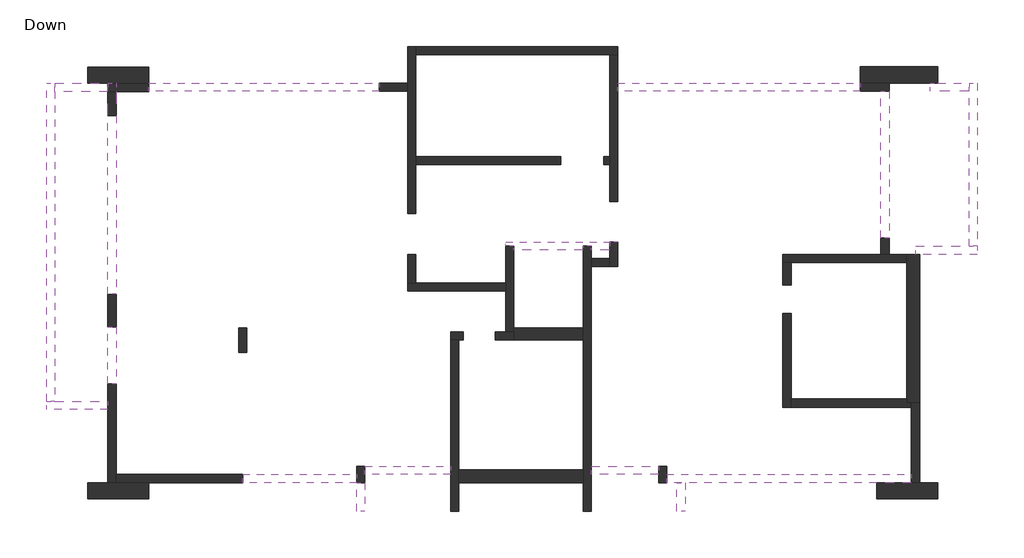
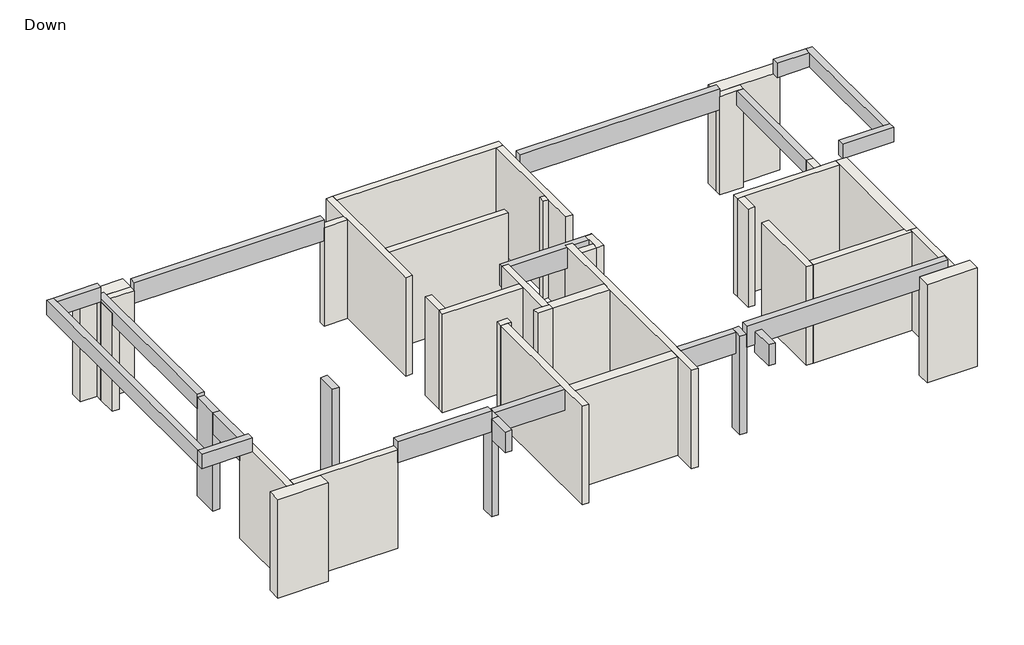
# One storey: 33 walls, 18 beams, 4 columns.
# Revit data of these elements (continued)
# Element 23 (IfcWall, "20") (continued)
#   SOFiSTiK_AMG_Comments = ""
#   Top Offset = 0 cm
#   Base Offset = 0 cm
#   wall height = 310 cm
#   SOFiSTiK_AMG_Scheduled = yes
#   SOFiSTiK_AMG_Adjusted = yes
#   Phase Created = New Construction
#   Base Constraint = Down
#   Top Constraint = Typical Floor
#   Materials on its faces: "Concrete"
# Element 24 (IfcWall, "20")
#   Comments = ""
#   Mark = "W6"
#   SOFiSTiK_EdgeZones = "W6"
#   SOFiSTiK_AMG_Comments = ""
#   Top Offset = 0 cm
#   Base Offset = 0 cm
#   wall height = 310 cm
#   SOFiSTiK_AMG_Scheduled = yes
#   SOFiSTiK_AMG_Adjusted = yes
#   Phase Created = New Construction
#   Base Constraint = Down
#   Top Constraint = Typical Floor
#   Materials on its faces: "Concrete"
# Element 25 (IfcWall, "20")
#   Comments = ""
#   Mark = "W7"
#   SOFiSTiK_EdgeZones = "W7"
#   SOFiSTiK_AMG_Comments = ""
#   Top Offset = 0 cm
#   Base Offset = 0 cm
#   wall height = 310 cm
#   SOFiSTiK_AMG_Scheduled = yes
#   SOFiSTiK_AMG_Adjusted = yes
#   Phase Created = New Construction
#   Base Constraint = Down
#   Top Constraint = Typical Floor
#   Materials on its faces: "Concrete"
# Element 26 (IfcWall, "20")
#   Comments = ""
#   Mark = "W8"
#   SOFiSTiK_EdgeZones = "W8"
#   SOFiSTiK_AMG_Comments = ""
#   Top Offset = 0 cm
#   Base Offset = 0 cm
#   wall height = 310 cm
#   SOFiSTiK_AMG_Scheduled = yes
#   SOFiSTiK_AMG_Adjusted = yes
#   Phase Created = New Construction
#   Base Constraint = Down
#   Top Constraint = Typical Floor
#   Materials on its faces: "Concrete"
# Element 27 (IfcWall, "20")
#   Comments = ""
#   Mark = "W9"
#   SOFiSTiK_EdgeZones = "W9"
#   SOFiSTiK_AMG_Comments = ""
#   Top Offset = 0 cm
#   Base Offset = 0 cm
#   wall height = 310 cm
#   SOFiSTiK_AMG_Scheduled = yes
#   SOFiSTiK_AMG_Adjusted = yes
#   Phase Created = New Construction
#   Base Constraint = Down
#   Top Constraint = Typical Floor
#   Materials on its faces: "Concrete"
# Element 28 (IfcWall, "20")
#   Comments = ""
#   Mark = "W10"
#   SOFiSTiK_EdgeZones = "W10"
#   SOFiSTiK_AMG_Comments = ""
#   Top Offset = 0 cm
#   Base Offset = 0 cm
#   wall height = 310 cm
#   SOFiSTiK_AMG_Scheduled = yes
#   SOFiSTiK_AMG_Adjusted = yes
#   Phase Created = New Construction
#   Base Constraint = Down
#   Top Constraint = Typical Floor
#   Materials on its faces: "Concrete"
# Element 29 (IfcWall, "20")
#   Comments = ""
#   Mark = "W11"
#   SOFiSTiK_EdgeZones = "W11"
#   SOFiSTiK_AMG_Comments = ""
#   Top Offset = 0 cm
#   Base Offset = 0 cm
#   wall height = 310 cm
#   SOFiSTiK_AMG_Scheduled = yes
#   SOFiSTiK_AMG_Adjusted = yes
#   Phase Created = New Construction
#   Base Constraint = Down
#   Top Constraint = Typical Floor
#   Materials on its faces: "Concrete"
# Element 30 (IfcWall, "20")
#   Comments = ""
#   Mark = "W12"
#   SOFiSTiK_EdgeZones = "W12"
#   SOFiSTiK_AMG_Comments = ""
#   Top Offset = 0 cm
#   Base Offset = 0 cm
#   wall height = 310 cm
#   SOFiSTiK_AMG_Scheduled = yes
#   SOFiSTiK_AMG_Adjusted = yes
#   Phase Created = New Construction
#   Base Constraint = Down
#   Top Constraint = Typical Floor
#   Materials on its faces: "Concrete"
# Element 31 (IfcWall, "20")
#   Comments = ""
#   Mark = "W13"
#   SOFiSTiK_EdgeZones = "W13"
#   SOFiSTiK_AMG_Comments = ""
#   Top Offset = 0 cm
#   Base Offset = 0 cm
#   wall height = 310 cm
#   SOFiSTiK_AMG_Scheduled = yes
#   SOFiSTiK_AMG_Adjusted = yes
#   Phase Created = New Construction
#   Base Constraint = Down
#   Top Constraint = Typical Floor
#   Materials on its faces: "Concrete"
# Element 32 (IfcWall, "20")
#   Comments = ""
#   Mark = "W14"
#   SOFiSTiK_EdgeZones = "W14"
#   SOFiSTiK_AMG_Comments = ""
#   Top Offset = 0 cm
#   Base Offset = 0 cm
#   wall height = 310 cm
#   SOFiSTiK_AMG_Scheduled = yes
#   SOFiSTiK_AMG_Adjusted = yes
#   Phase Created = New Construction
#   Base Constraint = Down
#   Top Constraint = Typical Floor
#   Materials on its faces: "Concrete"
# Element 33 (IfcWall, "20")
#   Comments = ""
#   Mark = "W16"
#   SOFiSTiK_EdgeZones = "W16"
#   SOFiSTiK_AMG_Comments = ""
#   Top Offset = 0 cm
#   Base Offset = 0 cm
#   wall height = 310 cm
#   SOFiSTiK_AMG_Scheduled = yes
#   SOFiSTiK_AMG_Adjusted = yes
#   Phase Created = New Construction
#   Base Constraint = Down
#   Top Constraint = Typical Floor
#   Materials on its faces: "Concrete"
# Element 34 (IfcWall, "20")
#   Comments = ""
#   Mark = "W17"
#   SOFiSTiK_EdgeZones = "W17"
#   SOFiSTiK_AMG_Comments = ""
#   Top Offset = 0 cm
#   Base Offset = 0 cm
#   wall height = 310 cm
#   SOFiSTiK_AMG_Scheduled = yes
#   SOFiSTiK_AMG_Adjusted = yes
#   Phase Created = New Construction
#   Base Constraint = Down
#   Top Constraint = Typical Floor
#   Materials on its faces: "Concrete"
# Element 35 (IfcWall, "20")
#   Comments = ""
#   Mark = "W18"
#   SOFiSTiK_EdgeZones = "W18"
#   SOFiSTiK_AMG_Comments = ""
#   Top Offset = 0 cm
#   Base Offset = 0 cm
#   wall height = 310 cm
#   SOFiSTiK_AMG_Scheduled = yes
#   SOFiSTiK_AMG_Adjusted = yes
#   Phase Created = New Construction
#   Base Constraint = Down
#   Top Constraint = Typical Floor
#   Materials on its faces: "Concrete"
# Element 36 (IfcWall, "20")
#   Comments = ""
#   Mark = "W19"
#   SOFiSTiK_EdgeZones = "W19"
#   SOFiSTiK_AMG_Comments = ""
#   Top Offset = 0 cm
#   Base Offset = 0 cm
#   wall height = 310 cm
#   SOFiSTiK_AMG_Scheduled = yes
#   SOFiSTiK_AMG_Adjusted = yes
#   Phase Created = New Construction
#   Base Constraint = Down
#   Top Constraint = Typical Floor
#   Materials on its faces: "Concrete"
# Element 37 (IfcWall, "20")
#   Comments = ""
#   Mark = "W20"
#   SOFiSTiK_EdgeZones = "W20"
#   SOFiSTiK_AMG_Comments = ""
#   Top Offset = 0 cm
#   Base Offset = 0 cm
#   wall height = 310 cm
#   SOFiSTiK_AMG_Scheduled = yes
#   SOFiSTiK_AMG_Adjusted = yes
#   Phase Created = New Construction
#   Base Constraint = Down
#   Top Constraint = Typical Floor
#   Materials on its faces: "Concrete"
# Element 38 (IfcWall, "20")
#   Comments = ""
#   Mark = "W21"
#   SOFiSTiK_EdgeZones = "W21"
#   SOFiSTiK_AMG_Comments = ""
#   Top Offset = 0 cm
#   Base Offset = 0 cm
#   wall height = 310 cm
#   SOFiSTiK_AMG_Scheduled = yes
#   SOFiSTiK_AMG_Adjusted = yes
#   Phase Created = New Construction
#   Base Constraint = Down
#   Top Constraint = Typical Floor
#   Materials on its faces: "Concrete"
# Element 39 (IfcWall, "20")
#   Comments = ""
#   Mark = "W22"
#   SOFiSTiK_EdgeZones = "W22"
#   SOFiSTiK_AMG_Comments = ""
#   Top Offset = 0 cm
#   Base Offset = 0 cm
#   wall height = 310 cm
#   SOFiSTiK_AMG_Scheduled = yes
#   SOFiSTiK_AMG_Adjusted = yes
#   Phase Created = New Construction
#   Base Constraint = Down
#   Top Constraint = Typical Floor
#   Materials on its faces: "Concrete"
# Element 40 (IfcWall, "20")
#   Comments = ""
#   Mark = "W23"
#   SOFiSTiK_EdgeZones = "W23"
#   SOFiSTiK_AMG_Comments = ""
#   Top Offset = 0 cm
#   Base Offset = 0 cm
#   wall height = 310 cm
#   SOFiSTiK_AMG_Scheduled = yes
#   SOFiSTiK_AMG_Adjusted = yes
#   Phase Created = New Construction
#   Base Constraint = Down
#   Top Constraint = Typical Floor
#   Materials on its faces: "Concrete"
# Element 41 (IfcWall, "20")
#   Comments = ""
#   Mark = "W24"
#   SOFiSTiK_EdgeZones = "W24"
#   SOFiSTiK_AMG_Comments = "Too Short /"
#   Top Offset = 0 cm
#   Base Offset = 0 cm
#   wall height = 310 cm
#   SOFiSTiK_AMG_Scheduled = yes
#   SOFiSTiK_AMG_Adjusted = yes
#   Phase Created = New Construction
#   Base Constraint = Down
#   Top Constraint = Typical Floor
#   Materials on its faces: "Concrete"
# Element 42 (IfcWall, "20")
#   Comments = ""
#   Mark = "W25"
#   SOFiSTiK_EdgeZones = "W25"
#   SOFiSTiK_AMG_Comments = ""
#   Top Offset = 0 cm
#   Base Offset = 0 cm
#   wall height = 310 cm
#   SOFiSTiK_AMG_Scheduled = yes
#   SOFiSTiK_AMG_Adjusted = yes
#   Phase Created = New Construction
#   Base Constraint = Down
#   Top Constraint = Typical Floor
#   Materials on its faces: "Concrete"
# Element 43 (IfcWall, "20")
#   Comments = ""
#   Mark = "W26"
#   SOFiSTiK_EdgeZones = "W26"
#   SOFiSTiK_AMG_Comments = ""
#   Top Offset = 0 cm
#   Base Offset = 0 cm
#   wall height = 310 cm
#   SOFiSTiK_AMG_Scheduled = yes
#   SOFiSTiK_AMG_Adjusted = yes
#   Phase Created = New Construction
#   Base Constraint = Down
#   Top Constraint = Typical Floor
#   Materials on its faces: "Concrete"
# Element 44 (IfcWall, "20")
#   Comments = ""
#   Mark = "W27"
#   SOFiSTiK_EdgeZones = "W27"
#   SOFiSTiK_AMG_Comments = ""
#   Top Offset = 0 cm
#   Base Offset = 0 cm
#   wall height = 310 cm
#   SOFiSTiK_AMG_Scheduled = yes
#   SOFiSTiK_AMG_Adjusted = yes
#   Phase Created = New Construction
#   Base Constraint = Down
#   Top Constraint = Typical Floor
#   Materials on its faces: "Concrete"
# Element 45 (IfcWall, "20")
#   Comments = ""
#   Mark = "W28"
#   SOFiSTiK_EdgeZones = "W28"
#   SOFiSTiK_AMG_Comments = ""
#   Top Offset = 0 cm
#   Base Offset = 0 cm
#   wall height = 310 cm
#   SOFiSTiK_AMG_Scheduled = yes
#   SOFiSTiK_AMG_Adjusted = yes
#   Phase Created = New Construction
#   Base Constraint = Down
#   Top Constraint = Typical Floor
#   Materials on its faces: "Concrete"
# Element 46 (IfcWall, "20")
#   Comments = ""
#   Mark = "W29"
#   SOFiSTiK_EdgeZones = "W29"
#   SOFiSTiK_AMG_Comments = ""
#   Top Offset = 0 cm
#   Base Offset = 0 cm
#   wall height = 310 cm
#   SOFiSTiK_AMG_Scheduled = yes
#   SOFiSTiK_AMG_Adjusted = yes
#   Phase Created = New Construction
#   Base Constraint = Down
#   Top Constraint = Typical Floor
#   Materials on its faces: "Concrete"
# Element 47 (IfcWall, "20")
#   Comments = ""
#   Mark = "W30"
#   SOFiSTiK_EdgeZones = "W30"
#   SOFiSTiK_AMG_Comments = ""
#   Top Offset = 0 cm
#   Base Offset = 0 cm
#   wall height = 310 cm
#   SOFiSTiK_AMG_Scheduled = yes
#   SOFiSTiK_AMG_Adjusted = yes
#   Phase Created = New Construction
#   Base Constraint = Down
#   Top Constraint = Typical Floor
#   Materials on its faces: "Concrete"
# Element 48 (IfcWall, "20")
#   Comments = ""
#   Mark = "W31"
#   SOFiSTiK_EdgeZones = "W31"
#   SOFiSTiK_AMG_Comments = ""
#   Top Offset = 0 cm
#   Base Offset = 0 cm
#   wall height = 310 cm
#   SOFiSTiK_AMG_Scheduled = yes
#   SOFiSTiK_AMG_Adjusted = yes
#   Phase Created = New Construction
#   Base Constraint = Down
#   Top Constraint = Typical Floor
#   Materials on its faces: "Concrete"
# Element 49 (IfcWall, "30")
#   Comments = ""
#   Mark = "W34"
#   SOFiSTiK_EdgeZones = "W34"
#   SOFiSTiK_AMG_Comments = ""
#   Top Offset = 0 cm
#   Base Offset = 0 cm
#   wall height = 310 cm
#   SOFiSTiK_AMG_Scheduled = yes
#   SOFiSTiK_AMG_Adjusted = yes
#   Phase Created = New Construction
#   Base Constraint = Down
#   Top Constraint = Typical Floor
#   Materials on its faces: "Concrete"
# Element 50 (IfcWall, "31")
#   Comments = ""
#   Mark = "W32"
#   SOFiSTiK_EdgeZones = "W32"
#   SOFiSTiK_AMG_Comments = ""
#   Top Offset = 0 cm
#   Base Offset = 0 cm
#   wall height = 310 cm
#   SOFiSTiK_AMG_Scheduled = yes
#   SOFiSTiK_AMG_Adjusted = yes
#   Phase Created = New Construction
#   Base Constraint = Down
#   Top Constraint = Typical Floor
#   Materials on its faces: "Concrete"
# Element 51 (IfcWall, "31")
#   Comments = ""
#   Mark = "W33"
#   SOFiSTiK_EdgeZones = "W33"
#   SOFiSTiK_AMG_Comments = ""
#   Top Offset = 0 cm
#   Base Offset = 0 cm
#   wall height = 310 cm
#   SOFiSTiK_AMG_Scheduled = yes
#   SOFiSTiK_AMG_Adjusted = yes
#   Phase Created = New Construction
#   Base Constraint = Down
#   Top Constraint = Typical Floor
#   Materials on its faces: "Concrete"
# Element 52 (IfcWall, "40")
#   Comments = ""
#   Mark = "W1"
#   SOFiSTiK_EdgeZones = "W1"
#   SOFiSTiK_AMG_Comments = ""
#   Top Offset = 0 cm
#   Base Offset = 0 cm
#   wall height = 310 cm
#   SOFiSTiK_AMG_Scheduled = yes
#   SOFiSTiK_AMG_Adjusted = yes
#   Phase Created = New Construction
#   Base Constraint = Down
#   Top Constraint = Typical Floor
#   Materials on its faces: "Concrete"
# Element 53 (IfcWall, "40")
#   Comments = ""
#   Mark = "W2"
#   SOFiSTiK_EdgeZones = "W2"
#   SOFiSTiK_AMG_Comments = ""
#   Top Offset = 0 cm
#   Base Offset = 0 cm
#   wall height = 310 cm
#   SOFiSTiK_AMG_Scheduled = yes
#   SOFiSTiK_AMG_Adjusted = yes
#   Phase Created = New Construction
#   Base Constraint = Down
#   Top Constraint = Typical Floor
#   Materials on its faces: "Concrete"
# Element 54 (IfcWall, "40")
#   Comments = ""
#   Mark = "W3"
#   SOFiSTiK_EdgeZones = "W3"
#   SOFiSTiK_AMG_Comments = ""
#   Top Offset = 0 cm
#   Base Offset = 0 cm
#   wall height = 310 cm
#   SOFiSTiK_AMG_Scheduled = yes
#   SOFiSTiK_AMG_Adjusted = yes
#   Phase Created = New Construction
#   Base Constraint = Down
#   Top Constraint = Typical Floor
#   Materials on its faces: "Concrete"
# Element 55 (IfcWall, "40")
#   Comments = ""
#   Mark = "W4"
#   SOFiSTiK_EdgeZones = "W4"
#   SOFiSTiK_AMG_Comments = ""
#   Top Offset = 0 cm
#   Base Offset = 0 cm
#   wall height = 310 cm
#   SOFiSTiK_AMG_Scheduled = yes
#   SOFiSTiK_AMG_Adjusted = yes
#   Phase Created = New Construction
#   Base Constraint = Down
#   Top Constraint = Typical Floor
#   Materials on its faces: "Concrete"
# Materials
#   "Concrete": class "Concrete", colour RGB 192 192 192, transparency 0, Keynote = "01000", Description = "Cast-in-place concrete", Cost = 0
